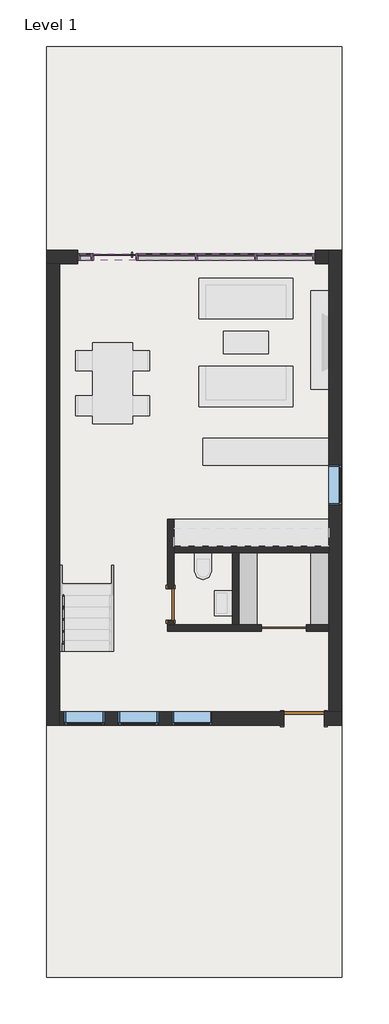
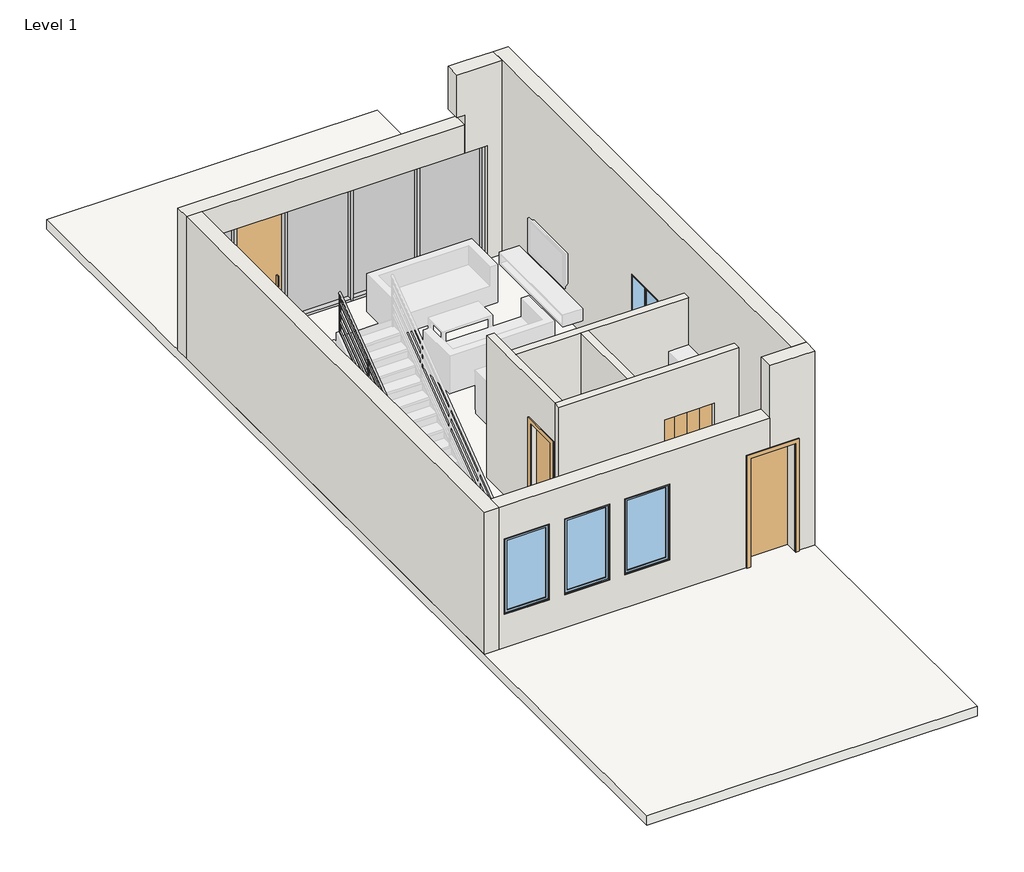
# One storey, part 1 of 2: 15 members, 10 walls, 4 doors, 4 plates, 4 windows, 1 railing, 1 slab.
"""IFC4 building model written with IfcOpenShell, lengths in millimetres."""

import ifcopenshell
import ifcopenshell.guid

model = None  # the IFC model being written
_history = None  # IfcOwnerHistory: only IFC2X3 demands one
_inside = {}  # id of a spatial element -> (the spatial element, [elements in it])
_under = {}  # id of a project, library or spatial element -> (it, [spatial elements below it])
_declared = {}  # id of a project -> (the project, [libraries it declares])
_typed = {}  # id of a type object -> (the type object, [elements of that type])
_made_of = {}  # id of a material, layer set ... -> (it, [elements and type objects made of it])


def new_model(schema):
    """Start an empty IFC model of exactly this schema.

    Asked for "IFC4X3", IfcOpenShell would pick the latest addendum, in which some entities
    have other attributes; the version numbers below select the first issue.
    IFC2X3 requires an IfcOwnerHistory on every rooted entity: one is made here for all.
    """
    global model, _history
    if schema == "IFC4X3":
        model = ifcopenshell.file(schema_version=(4, 3, 0, 0))
    else:
        model = ifcopenshell.file(schema=schema)
    _inside.clear()
    _under.clear()
    _declared.clear()
    _typed.clear()
    _made_of.clear()
    _history = None
    if model.schema == "IFC2X3":
        org = make("IfcOrganization", Name="unknown")
        user = make(
            "IfcPersonAndOrganization",
            ThePerson=make("IfcPerson", FamilyName="unknown"),
            TheOrganization=org,
        )
        app = make(
            "IfcApplication",
            ApplicationDeveloper=org,
            Version="unknown",
            ApplicationFullName="unknown",
            ApplicationIdentifier="unknown",
        )
        _history = make(
            "IfcOwnerHistory",
            OwningUser=user,
            OwningApplication=app,
            ChangeAction="ADDED",
            CreationDate=0,
        )
    return model


def make(cls, **values):
    """One entity of the class cls with the attributes given. An attribute that is None is left unset."""
    return model.create_entity(
        cls, **{name: value for name, value in values.items() if value is not None}
    )


def rooted(cls, **values):
    """An entity with a GlobalId (a new one), such as an element, a storey or a relation."""
    return make(cls, GlobalId=ifcopenshell.guid.new(), OwnerHistory=_history, **values)


def si_unit(unit_type, name, prefix=None):
    """IfcSIUnit, for example si_unit("LENGTHUNIT", "METRE", prefix="MILLI")."""
    return make("IfcSIUnit", UnitType=unit_type, Prefix=prefix, Name=name)


def assignment(units):
    """IfcUnitAssignment: the units of a project."""
    return None if units is None else make("IfcUnitAssignment", Units=units)


def point(xyz):
    """IfcCartesianPoint."""
    return None if xyz is None else make("IfcCartesianPoint", Coordinates=xyz)


def direction(xyz):
    """IfcDirection."""
    return None if xyz is None else make("IfcDirection", DirectionRatios=xyz)


def frame(location, z_axis=None, x_axis=None):
    """IfcAxis2Placement3D, a coordinate frame: its origin and axes. An axis left out is left unset."""
    return make(
        "IfcAxis2Placement3D",
        Location=point(location),
        Axis=direction(z_axis),
        RefDirection=direction(x_axis),
    )


def origin():
    """The frame at (0, 0, 0) with its axes left unset."""
    return frame((0.0, 0.0, 0.0))


def origin_with_axes():
    """The frame at (0, 0, 0) with the z axis (0, 0, 1) and the x axis (1, 0, 0) written out."""
    return frame((0.0, 0.0, 0.0), z_axis=(0.0, 0.0, 1.0), x_axis=(1.0, 0.0, 0.0))


def place(relative_to, where):
    """IfcLocalPlacement: puts the frame where relative to a parent placement (None: the world)."""
    return make(
        "IfcLocalPlacement", PlacementRelTo=relative_to, RelativePlacement=where
    )


def context(
    kind, dimensions, precision=None, world=None, true_north=None, identifier=None
):
    """IfcGeometricRepresentationContext, for example the 3D "Model" context."""
    return make(
        "IfcGeometricRepresentationContext",
        ContextIdentifier=identifier,
        ContextType=kind,
        CoordinateSpaceDimension=dimensions,
        Precision=precision,
        WorldCoordinateSystem=world,
        TrueNorth=true_north,
    )


def project(units=None, contexts=None):
    """IfcProject with its units and contexts."""
    return rooted(
        "IfcProject",
        Name="project",
        RepresentationContexts=contexts,
        UnitsInContext=assignment(units),
    )


def spatial(cls, under=None, at=None, **own):
    """A site, building, storey or space (cls), placed at a placement, below another one or the project."""
    s = rooted(cls, ObjectPlacement=at, **own)
    if under is not None:
        _under.setdefault(under.id(), (under, []))[1].append(s)
    return s


def polyline(points):
    """IfcPolyline through the points."""
    return make("IfcPolyline", Points=[point(p) for p in points])


def circle_curve(where, radius):
    """IfcCircle in the frame where."""
    return make("IfcCircle", Position=where, Radius=radius)


def ellipse_curve(where, semi_axis1, semi_axis2):
    """IfcEllipse in the frame where."""
    return make(
        "IfcEllipse", Position=where, SemiAxis1=semi_axis1, SemiAxis2=semi_axis2
    )


def outline(outer, holes=None, kind="AREA"):
    """IfcArbitraryClosedProfileDef: a profile drawn as a closed curve; with holes, ...WithVoids."""
    if holes is None:
        return make("IfcArbitraryClosedProfileDef", ProfileType=kind, OuterCurve=outer)
    return make(
        "IfcArbitraryProfileDefWithVoids",
        ProfileType=kind,
        OuterCurve=outer,
        InnerCurves=holes,
    )


def extrude(swept, where, along, depth):
    """IfcExtrudedAreaSolid: the profile swept, set in the frame where, extruded along a direction by depth."""
    return make(
        "IfcExtrudedAreaSolid",
        SweptArea=swept,
        Position=where,
        ExtrudedDirection=direction(along),
        Depth=depth,
    )


def faces_of(points, faces, orient=None, outer=None):
    """IfcFace entities. A face is a list of loops; a loop is a list of indices into points, from 0.

    orient and outer hold one flag for each loop. By default every Orientation is true, the
    first loop of a face is its IfcFaceOuterBound and the others are IfcFaceBound.
    """
    made = []
    for i, loops in enumerate(faces):
        bounds = []
        for j, loop in enumerate(loops):
            is_outer = j == 0 if outer is None else outer[i][j]
            bounds.append(
                make(
                    "IfcFaceOuterBound" if is_outer else "IfcFaceBound",
                    Bound=make("IfcPolyLoop", Polygon=[points[k] for k in loop]),
                    Orientation=True if orient is None else orient[i][j],
                )
            )
        made.append(make("IfcFace", Bounds=bounds))
    return made


def faceted_brep(points, faces, orient=None, outer=None, voids=None):
    """IfcFacetedBrep: a solid bounded by flat faces; with voids (closed shells), ...WithVoids."""
    shared = [point(p) for p in points]
    hull = make("IfcClosedShell", CfsFaces=faces_of(shared, faces, orient, outer))
    if voids is None:
        return make("IfcFacetedBrep", Outer=hull)
    return make(
        "IfcFacetedBrepWithVoids",
        Outer=hull,
        Voids=[
            make(cls, CfsFaces=faces_of(shared, fs, o, b)) for cls, fs, o, b in voids
        ],
    )


def shape(context_of_items, identifier, shape_type, items):
    """IfcShapeRepresentation: the items that make up one representation, for example the "Body"."""
    return make(
        "IfcShapeRepresentation",
        ContextOfItems=context_of_items,
        RepresentationIdentifier=identifier,
        RepresentationType=shape_type,
        Items=items,
    )


def source(mapping_origin, context_of_items, identifier, shape_type, items):
    """IfcRepresentationMap: a shape defined once, which mapped items show again and again."""
    return make(
        "IfcRepresentationMap",
        MappingOrigin=mapping_origin,
        MappedRepresentation=shape(context_of_items, identifier, shape_type, items),
    )


def transform(
    local_origin,
    x_axis=None,
    y_axis=None,
    z_axis=None,
    scale=None,
    scale2=None,
    scale3=None,
    uniform=True,
):
    """IfcCartesianTransformationOperator3D, or its non-uniform kind. x_axis, y_axis, z_axis: its Axis1, 2, 3."""
    if uniform:
        return make(
            "IfcCartesianTransformationOperator3D",
            Axis1=direction(x_axis),
            Axis2=direction(y_axis),
            LocalOrigin=point(local_origin),
            Scale=scale,
            Axis3=direction(z_axis),
        )
    return make(
        "IfcCartesianTransformationOperator3DnonUniform",
        Axis1=direction(x_axis),
        Axis2=direction(y_axis),
        LocalOrigin=point(local_origin),
        Scale=scale,
        Axis3=direction(z_axis),
        Scale2=scale2,
        Scale3=scale3,
    )


def mapped(mapping_source, mapping_target):
    """IfcMappedItem: shows the shape of a source again, moved by a transform."""
    return make(
        "IfcMappedItem", MappingSource=mapping_source, MappingTarget=mapping_target
    )


def made_of(thing, what):
    """Note that an element or type object is made of a material, layer set ...; save() writes the relation."""
    if what is not None:
        _made_of.setdefault(what.id(), (what, []))[1].append(thing)
    return thing


def element(
    cls,
    number,
    at=None,
    inside=None,
    cuts=None,
    type_object=None,
    material=None,
    context=None,
    identifier="Body",
    shape_type=None,
    held_by="IfcProductDefinitionShape",
    body=None,
    shapes=None,
    **own,
):
    """One element of the class cls, such as IfcWall. Its Tag is "e" and its number.

    at: its placement. inside: the storey or other place that contains it. cuts: it is an
    opening in that element (IfcRelVoidsElement). A single representation is given by context,
    identifier, shape_type and body (its items); several are given by shapes. held_by: the class
    of the entity that holds the representations. save() writes the other relations.
    """
    e = rooted(cls, Tag="e%d" % number, ObjectPlacement=at, **own)
    if body is not None:
        shapes = [shape(context, identifier, shape_type, body)]
    if shapes is not None:
        e.Representation = make(held_by, Representations=shapes)
    if inside is not None:
        _inside.setdefault(inside.id(), (inside, []))[1].append(e)
    if cuts is not None:
        rooted(
            "IfcRelVoidsElement", RelatingBuildingElement=cuts, RelatedOpeningElement=e
        )
    if type_object is not None:
        _typed.setdefault(type_object.id(), (type_object, []))[1].append(e)
    return made_of(e, material)


def aggregate(whole, parts):
    """IfcRelAggregates: a whole, such as a stair, and the parts it consists of."""
    return rooted("IfcRelAggregates", RelatingObject=whole, RelatedObjects=parts)


def save(model, path):
    """Write the relations noted so far, then the file.

    IfcRelAggregates (storeys below a building ...), IfcRelContainedInSpatialStructure (elements
    in a storey), IfcRelDefinesByType, IfcRelAssociatesMaterial and IfcRelDeclares: one each for
    every whole, place, type object, material and project.
    """
    for whole, parts in _under.values():
        aggregate(whole, parts)
    for where, things in _inside.values():
        rooted(
            "IfcRelContainedInSpatialStructure",
            RelatedElements=things,
            RelatingStructure=where,
        )
    for kind, things in _typed.values():
        rooted("IfcRelDefinesByType", RelatedObjects=things, RelatingType=kind)
    for what, things in _made_of.values():
        rooted("IfcRelAssociatesMaterial", RelatedObjects=things, RelatingMaterial=what)
    for by, libraries in _declared.values():
        rooted("IfcRelDeclares", RelatingContext=by, RelatedDefinitions=libraries)
    model.write(path)


def plane_surface(at):
    """IfcPlane: the flat surface through the origin of the frame at, square to its z axis."""
    return make("IfcPlane", Position=at)


def cylinder_surface(at, radius):
    """IfcCylindricalSurface: all points at the distance radius from the z axis of the frame at."""
    return make("IfcCylindricalSurface", Position=at, Radius=radius)


def advanced_brep(points, edges, surfaces, faces):
    """IfcAdvancedBrep: a solid bounded by faces that lie on surfaces and meet in shared edges.

    An edge is (start, end): straight between two places in points (the first is 0);
    or (start, end, curve); or (start, end, curve, False) where it runs against its curve.
    A face is (place in surfaces, loops), or (place, loops, False) where it looks against
    its surface's normal. A loop lists edges by number (the first is 1), with a minus sign
    where the edge is run from its end to its start. The first loop is the outer one.
    """
    corners = [point(p) for p in points]
    vertices = [make("IfcVertexPoint", VertexGeometry=c) for c in corners]
    made = []
    for start, end, *more in edges:
        made.append(
            make(
                "IfcEdgeCurve",
                EdgeStart=vertices[start],
                EdgeEnd=vertices[end],
                EdgeGeometry=more[0] if more else make("IfcPolyline", Points=[corners[start], corners[end]]),
                SameSense=more[1] if len(more) > 1 else True,
            )
        )
    hull = []
    for where, loops, *sense in faces:
        bounds = []
        for j, loop in enumerate(loops):
            ring = [make("IfcOrientedEdge", EdgeElement=made[abs(k) - 1], Orientation=k > 0) for k in loop]
            bounds.append(
                make(
                    "IfcFaceOuterBound" if j == 0 else "IfcFaceBound",
                    Bound=make("IfcEdgeLoop", EdgeList=ring),
                    Orientation=True,
                )
            )
        hull.append(make("IfcAdvancedFace", Bounds=bounds, FaceSurface=surfaces[where], SameSense=sense[0] if sense else True))
    return make("IfcAdvancedBrep", Outer=make("IfcClosedShell", CfsFaces=hull))


def door_88445510(model_context):
    return source(origin(), model_context, "Body", "SweptSolid", [
        extrude(outline(polyline([(255.0, 10.0), (500.0, 10.0), (500.0, -10.0), (-500.0, -10.0), (-500.0, 10.0), (-255.0, 10.0), (-255.0, 0.0), (-245.0, 0.0), (-245.0, 10.0), (-5.0, 10.0), (-5.0, 0.0), (5.0, 0.0), (5.0, 10.0), (245.0, 10.0), (245.0, 0.0), (255.0, 0.0), (255.0, 10.0)])), origin_with_axes(), (0.0, 0.0, 1.0), 2000.0),
    ])


def ba_basic_door_70_x_210cm_b6d038f8(model_context):
    return source(origin(), model_context, "Body", "SweptSolid", [
        extrude(outline(polyline([(350.0, 24.0), (-350.0, 24.0), (-350.0, 75.0), (350.0, 75.0), (350.0, 24.0)])), origin_with_axes(), (0.0, 0.0, 1.0), 2100.0),
        extrude(outline(polyline([(2176.0, -426.0), (0.0, -426.0), (0.0, -350.0), (2100.0, -350.0), (2100.0, 350.0), (0.0, 350.0), (0.0, 426.0), (2176.0, 426.0), (2176.0, -426.0)])), frame((0.0, 75.0, 0.0), z_axis=(0.0, 1.0, 0.0), x_axis=(0.0, 0.0, 1.0)), (0.0, 0.0, 1.0), 25.0),
        extrude(outline(polyline([(2176.0, 426.0), (2176.0, -426.0), (0.0, -426.0), (0.0, -350.0), (2100.0, -350.0), (2100.0, 350.0), (0.0, 350.0), (0.0, 426.0), (2176.0, 426.0)])), frame((0.0, -100.0, 0.0), z_axis=(0.0, 1.0, 0.0), x_axis=(0.0, 0.0, 1.0)), (0.0, 0.0, 1.0), 25.0),
    ])


def ba_basic_door_90_x_230cm_e5931120(model_context):
    return source(origin(), model_context, "Body", "SweptSolid", [
        extrude(outline(polyline([(450.0, 99.0), (-450.0, 99.0), (-450.0, 150.0), (450.0, 150.0), (450.0, 99.0)])), origin_with_axes(), (0.0, 0.0, 1.0), 2300.0),
        extrude(outline(polyline([(2376.0, -526.0), (0.0, -526.0), (0.0, -450.0), (2300.0, -450.0), (2300.0, 450.0), (0.0, 450.0), (0.0, 526.0), (2376.0, 526.0), (2376.0, -526.0)])), frame((0.0, 150.0, 0.0), z_axis=(0.0, 1.0, 0.0), x_axis=(0.0, 0.0, 1.0)), (0.0, 0.0, 1.0), 25.0),
        extrude(outline(polyline([(2376.0, 526.0), (2376.0, -526.0), (0.0, -526.0), (0.0, -450.0), (2300.0, -450.0), (2300.0, 450.0), (0.0, 450.0), (0.0, 526.0), (2376.0, 526.0)])), frame((0.0, -175.0, 0.0), z_axis=(0.0, 1.0, 0.0), x_axis=(0.0, 0.0, 1.0)), (0.0, 0.0, 1.0), 25.0),
    ])


def m_door_curtain_wall_single_glass_m_door_curtain_wall_single_99f07895(model_context):
    return source(origin(), model_context, "Body", "SweptSolid", [
        extrude(outline(polyline([(475.0, -50.8), (-475.0, -50.8), (-475.0, -38.1), (475.0, -38.1), (475.0, -50.8)])), origin_with_axes(), (0.0, 0.0, 1.0), 2350.0),
        extrude(outline(polyline([(-373.4, 12.7), (-373.4, -38.1), (-398.8, -38.1), (-398.8, 12.7), (-373.4, 12.7)])), frame((0.0, 0.0, 762.0), z_axis=(0.0, 0.0, 1.0), x_axis=(1.0, 0.0, 0.0)), (0.0, 0.0, 1.0), 228.6),
        extrude(outline(polyline([(-398.8, -101.6), (-398.8, -50.8), (-373.4, -50.8), (-373.4, -101.6), (-398.8, -101.6)])), frame((0.0, 0.0, 762.0), z_axis=(0.0, 0.0, 1.0), x_axis=(1.0, 0.0, 0.0)), (0.0, 0.0, 1.0), 228.6),
    ])


def rectangular_mullion_50_x_150mm_8d7ec0e8(model_context):
    return source(origin(), model_context, "Body", "SweptSolid", [
        extrude(outline(polyline([(0.0, 75.0), (0.0, -75.0), (-50.0, -75.0), (-50.0, 75.0), (0.0, 75.0)])), frame((0.0, 0.0, -1250.0000002), z_axis=(0.0, 0.0, 1.0), x_axis=(1.0, 0.0, 0.0)), (0.0, 0.0, 1.0), 1250.0000002),
    ])


def rectangular_mullion_50_x_150mm_345eee08(model_context):
    return source(origin(), model_context, "Body", "SweptSolid", [
        extrude(outline(polyline([(0.0, 75.0), (0.0, -75.0), (-50.0, -75.0), (-50.0, 75.0), (0.0, 75.0)])), frame((0.0, 0.0, -1274.9999998), z_axis=(0.0, 0.0, 1.0), x_axis=(1.0, 0.0, 0.0)), (0.0, 0.0, 1.0), 1274.9999998),
    ])


def rectangular_mullion_50_x_150mm_6225e4e3(model_context):
    return source(origin(), model_context, "Body", "SweptSolid", [
        extrude(outline(polyline([(25.0, 75.0), (25.0, -75.0), (-25.0, -75.0), (-25.0, 75.0), (25.0, 75.0)])), frame((0.0, 0.0, -2400.0), z_axis=(0.0, 0.0, 1.0), x_axis=(1.0, 0.0, 0.0)), (0.0, 0.0, 1.0), 2400.0),
    ])


def rectangular_mullion_50_x_150mm_662c37b1(model_context):
    return source(origin(), model_context, "Body", "SweptSolid", [
        extrude(outline(polyline([(0.0, 75.0), (0.0, -75.0), (-50.0, -75.0), (-50.0, 75.0), (0.0, 75.0)])), frame((0.0, 0.0, -2400.0), z_axis=(0.0, 0.0, 1.0), x_axis=(1.0, 0.0, 0.0)), (0.0, 0.0, 1.0), 2400.0),
    ])


def rectangular_mullion_50_x_150mm_12a430f9(model_context):
    return source(origin(), model_context, "Body", "SweptSolid", [
        extrude(outline(polyline([(0.0, 75.0), (0.0, -75.0), (-50.0, -75.0), (-50.0, 75.0), (0.0, 75.0)])), frame((0.0, 0.0, -950.0), z_axis=(0.0, 0.0, 1.0), x_axis=(1.0, 0.0, 0.0)), (0.0, 0.0, 1.0), 950.0),
    ])


def rectangular_mullion_50_x_150mm_43431b2b(model_context):
    return source(origin(), model_context, "Body", "SweptSolid", [
        extrude(outline(polyline([(0.0, 75.0), (0.0, -75.0), (-50.0, -75.0), (-50.0, 75.0), (0.0, 75.0)])), frame((0.0, 0.0, -250.0000002), z_axis=(0.0, 0.0, 1.0), x_axis=(1.0, 0.0, 0.0)), (0.0, 0.0, 1.0), 250.0000002),
    ])


def system_panel_glazed_960e6087(model_context):
    return source(origin(), model_context, "Body", "SweptSolid", [
        extrude(outline(polyline([(625.0000001, 24.5), (-625.0000001, 24.5), (-625.0000001, 49.5), (625.0000001, 49.5), (625.0000001, 24.5)])), origin_with_axes(), (0.0, 0.0, 1.0), 2300.0),
    ])


def system_panel_glazed_939e179a(model_context):
    return source(origin(), model_context, "Body", "SweptSolid", [
        extrude(outline(polyline([(637.4999999, 24.5), (-637.4999999, 24.5), (-637.4999999, 49.5), (637.4999999, 49.5), (637.4999999, 24.5)])), origin_with_axes(), (0.0, 0.0, 1.0), 2300.0),
    ])


def system_panel_glazed_27ab1db5(model_context):
    return source(origin(), model_context, "Body", "SweptSolid", [
        extrude(outline(polyline([(125.0000001, 24.5), (-125.0000001, 24.5), (-125.0000001, 49.5), (125.0000001, 49.5), (125.0000001, 24.5)])), origin_with_axes(), (0.0, 0.0, 1.0), 2300.0),
    ])


def ba_window_900_x_1600mm_2_0de2e490(model_context):
    return source(origin(), model_context, "Body", "SweptSolid", [
        extrude(outline(polyline([(-387.0, 128.0), (387.0, 128.0), (387.0, 116.0), (-387.0, 116.0), (-387.0, 128.0)])), frame((0.0, 0.0, 978.0), z_axis=(0.0, 0.0, 1.0), x_axis=(1.0, 0.0, 0.0)), (0.0, 0.0, 1.0), 1474.0),
        extrude(outline(polyline([(2496.0, -431.0), (934.0, -431.0), (934.0, 431.0), (2496.0, 431.0), (2496.0, -431.0)]), holes=[polyline([(2452.0, -387.0), (2452.0, 387.0), (978.0, 387.0), (978.0, -387.0), (2452.0, -387.0)])]), frame((0.0, 100.0, 0.0), z_axis=(0.0, 1.0, 0.0), x_axis=(0.0, 0.0, 1.0)), (0.0, 0.0, 1.0), 44.0),
        extrude(outline(polyline([(2515.0, -450.0), (915.0, -450.0), (915.0, 450.0), (2515.0, 450.0), (2515.0, -450.0)]), holes=[polyline([(2496.0, -431.0), (2496.0, 431.0), (934.0, 431.0), (934.0, -431.0), (2496.0, -431.0)])]), frame((0.0, 100.0, 0.0), z_axis=(0.0, 1.0, 0.0), x_axis=(0.0, 0.0, 1.0)), (0.0, 0.0, 1.0), 63.0),
        extrude(outline(polyline([(2515.0, -450.0), (915.0, -450.0), (915.0, 450.0), (2515.0, 450.0), (2515.0, -450.0)]), holes=[polyline([(2483.0, -418.0), (2483.0, 418.0), (947.0, 418.0), (947.0, -418.0), (2483.0, -418.0)])]), frame((0.0, -137.0, 0.0), z_axis=(0.0, 1.0, 0.0), x_axis=(0.0, 0.0, 1.0)), (0.0, 0.0, 1.0), 237.0),
    ])


def ba_window_900_x_1600mm_2_f3ed7943(model_context):
    return source(origin(), model_context, "Body", "SweptSolid", [
        extrude(outline(polyline([(-387.0, -128.0), (-387.0, -116.0), (387.0, -116.0), (387.0, -128.0), (-387.0, -128.0)])), frame((0.0, 0.0, 978.0), z_axis=(0.0, 0.0, 1.0), x_axis=(1.0, 0.0, 0.0)), (0.0, 0.0, 1.0), 1474.0),
        extrude(outline(polyline([(2496.0, -431.0), (934.0, -431.0), (934.0, 431.0), (2496.0, 431.0), (2496.0, -431.0)]), holes=[polyline([(2452.0, -387.0), (2452.0, 387.0), (978.0, 387.0), (978.0, -387.0), (2452.0, -387.0)])]), frame((0.0, -144.0, 0.0), z_axis=(0.0, 1.0, 0.0), x_axis=(0.0, 0.0, 1.0)), (0.0, 0.0, 1.0), 44.0),
        extrude(outline(polyline([(2515.0, -450.0), (915.0, -450.0), (915.0, 450.0), (2515.0, 450.0), (2515.0, -450.0)]), holes=[polyline([(2496.0, -431.0), (2496.0, 431.0), (934.0, 431.0), (934.0, -431.0), (2496.0, -431.0)])]), frame((0.0, -163.0, 0.0), z_axis=(0.0, 1.0, 0.0), x_axis=(0.0, 0.0, 1.0)), (0.0, 0.0, 1.0), 63.0),
        extrude(outline(polyline([(2515.0, -450.0), (915.0, -450.0), (915.0, 450.0), (2515.0, 450.0), (2515.0, -450.0)]), holes=[polyline([(2483.0, -418.0), (2483.0, 418.0), (947.0, 418.0), (947.0, -418.0), (2483.0, -418.0)])]), frame((0.0, -100.0, 0.0), z_axis=(0.0, 1.0, 0.0), x_axis=(0.0, 0.0, 1.0)), (0.0, 0.0, 1.0), 237.0),
    ])


model = new_model("IFC4")

# Units and contexts
model_context = context("Model", 3, world=origin())
ifc_project = project(units=[si_unit("LENGTHUNIT", "METRE", prefix="MILLI")], contexts=[model_context])

# Site, building, storey
site = spatial("IfcSite", under=ifc_project)
building = spatial("IfcBuilding", under=site)
storey = spatial("IfcBuildingStorey", under=building, Name="Level 1", Elevation=0.0)

# Doors
placement = place(None, origin())
door_shape = door_88445510(model_context)
element("IfcDoor", 1, ObjectType="BA_Bi-fold door : AD_Bi-fold door - 100cm", at=placement, inside=storey, context=model_context, shape_type="MappedRepresentation", body=[
    mapped(door_shape, transform((2017.9856921, -6579.202269, 0.0), x_axis=(-1.0, 0.0, 0.0), y_axis=(0.0, -1.0, 0.0), z_axis=(0.0, 0.0, 1.0))),
])
ba_basic_door_70_x_210cm_shape = ba_basic_door_70_x_210cm_b6d038f8(model_context)
element("IfcDoor", 2, ObjectType="BA_Basic Door : 70 x 210cm", at=placement, inside=storey, context=model_context, shape_type="MappedRepresentation", body=[
    mapped(ba_basic_door_70_x_210cm_shape, transform((-507.0143079, -6054.202269, 0.0), x_axis=(0.0, -1.0, 0.0), y_axis=(1.0, 0.0, 0.0), z_axis=(0.0, 0.0, 1.0))),
])
ba_basic_door_90_x_230cm_shape = ba_basic_door_90_x_230cm_e5931120(model_context)
element("IfcDoor", 3, ObjectType="BA_Basic Door : 90 x 230cm", at=placement, inside=storey, context=model_context, shape_type="MappedRepresentation", body=[
    mapped(ba_basic_door_90_x_230cm_shape, transform((2467.9856921, -8604.202269, 0.0), x_axis=(1.0, 0.0, 0.0), y_axis=(0.0, 1.0, 0.0), z_axis=(0.0, 0.0, 1.0))),
])
m_door_curtain_wall_single_glass_m_door_curtain_wall_single_shape = m_door_curtain_wall_single_glass_m_door_curtain_wall_single_99f07895(model_context)
element("IfcDoor", 4, ObjectType="M_Door-Curtain-Wall-Single-Glass : M_Door-Curtain-Wall-Single-Glass", at=placement, inside=storey, context=model_context, shape_type="MappedRepresentation", body=[
    mapped(m_door_curtain_wall_single_glass_m_door_curtain_wall_single_shape, transform((-1757.0143078, 1695.797731, 0.0), x_axis=(-1.0, 0.0, 0.0), y_axis=(0.0, -1.0, 0.0), z_axis=(0.0, 0.0, 1.0))),
])

# Members
rectangular_mullion_50_x_150mm_shape = rectangular_mullion_50_x_150mm_8d7ec0e8(model_context)
element("IfcMember", 5, ObjectType="Rectangular Mullion : 50 x 150mm", at=placement, inside=storey, context=model_context, shape_type="MappedRepresentation", body=[
    mapped(rectangular_mullion_50_x_150mm_shape, transform((2667.9856921, 1695.797731, 2400.0), x_axis=(0.0, 0.0, 1.0), y_axis=(0.0, -1.0, 0.0), z_axis=(1.0, 0.0, 0.0))),
])
rectangular_mullion_50_x_150mm_2_shape = rectangular_mullion_50_x_150mm_345eee08(model_context)
element("IfcMember", 6, ObjectType="Rectangular Mullion : 50 x 150mm", at=placement, inside=storey, context=model_context, shape_type="MappedRepresentation", body=[
    mapped(rectangular_mullion_50_x_150mm_2_shape, transform((42.9856921, 1695.797731, 2400.0), x_axis=(0.0, 0.0, 1.0), y_axis=(0.0, -1.0, 0.0), z_axis=(1.0, 0.0, 0.0))),
])
element("IfcMember", 7, ObjectType="Rectangular Mullion : 50 x 150mm", at=placement, inside=storey, context=model_context, shape_type="MappedRepresentation", body=[
    mapped(rectangular_mullion_50_x_150mm_2_shape, transform((1367.9856919, 1695.797731, 2400.0), x_axis=(0.0, 0.0, 1.0), y_axis=(0.0, -1.0, 0.0), z_axis=(1.0, 0.0, 0.0))),
])
element("IfcMember", 8, ObjectType="Rectangular Mullion : 50 x 150mm", at=placement, inside=storey, context=model_context, shape_type="MappedRepresentation", body=[
    mapped(rectangular_mullion_50_x_150mm_shape, transform((1417.9856919, 1695.797731, 0.0), x_axis=(0.0, 0.0, -1.0), y_axis=(0.0, -1.0, 0.0), z_axis=(-1.0, 0.0, 0.0))),
])
element("IfcMember", 9, ObjectType="Rectangular Mullion : 50 x 150mm", at=placement, inside=storey, context=model_context, shape_type="MappedRepresentation", body=[
    mapped(rectangular_mullion_50_x_150mm_2_shape, transform((-1232.0143078, 1695.797731, 0.0), x_axis=(0.0, 0.0, -1.0), y_axis=(0.0, -1.0, 0.0), z_axis=(-1.0, 0.0, 0.0))),
])
element("IfcMember", 10, ObjectType="Rectangular Mullion : 50 x 150mm", at=placement, inside=storey, context=model_context, shape_type="MappedRepresentation", body=[
    mapped(rectangular_mullion_50_x_150mm_2_shape, transform((92.9856921, 1695.797731, 0.0), x_axis=(0.0, 0.0, -1.0), y_axis=(0.0, -1.0, 0.0), z_axis=(-1.0, 0.0, 0.0))),
])
rectangular_mullion_50_x_150mm_3_shape = rectangular_mullion_50_x_150mm_6225e4e3(model_context)
element("IfcMember", 11, ObjectType="Rectangular Mullion : 50 x 150mm", at=placement, inside=storey, context=model_context, shape_type="MappedRepresentation", body=[
    mapped(rectangular_mullion_50_x_150mm_3_shape, transform((-1257.0143078, 1695.797731, 0.0), x_axis=(1.0, 0.0, 0.0), y_axis=(0.0, -1.0, 0.0), z_axis=(0.0, 0.0, -1.0))),
])
element("IfcMember", 12, ObjectType="Rectangular Mullion : 50 x 150mm", at=placement, inside=storey, context=model_context, shape_type="MappedRepresentation", body=[
    mapped(rectangular_mullion_50_x_150mm_3_shape, transform((67.9856921, 1695.797731, 0.0), x_axis=(1.0, 0.0, 0.0), y_axis=(0.0, -1.0, 0.0), z_axis=(0.0, 0.0, -1.0))),
])
element("IfcMember", 13, ObjectType="Rectangular Mullion : 50 x 150mm", at=placement, inside=storey, context=model_context, shape_type="MappedRepresentation", body=[
    mapped(rectangular_mullion_50_x_150mm_3_shape, transform((1392.9856919, 1695.797731, 0.0), x_axis=(1.0, 0.0, 0.0), y_axis=(0.0, -1.0, 0.0), z_axis=(0.0, 0.0, -1.0))),
])
element("IfcMember", 14, ObjectType="Rectangular Mullion : 50 x 150mm", at=placement, inside=storey, context=model_context, shape_type="MappedRepresentation", body=[
    mapped(rectangular_mullion_50_x_150mm_3_shape, transform((-2257.0143078, 1695.797731, 0.0), x_axis=(1.0, 0.0, 0.0), y_axis=(0.0, -1.0, 0.0), z_axis=(0.0, 0.0, -1.0))),
])
rectangular_mullion_50_x_150mm_4_shape = rectangular_mullion_50_x_150mm_662c37b1(model_context)
element("IfcMember", 15, ObjectType="Rectangular Mullion : 50 x 150mm", at=placement, inside=storey, context=model_context, shape_type="MappedRepresentation", body=[
    mapped(rectangular_mullion_50_x_150mm_4_shape, transform((2717.9856921, 1695.797731, 0.0), x_axis=(1.0, 0.0, 0.0), y_axis=(0.0, -1.0, 0.0), z_axis=(0.0, 0.0, -1.0))),
])
element("IfcMember", 16, ObjectType="Rectangular Mullion : 50 x 150mm", at=placement, inside=storey, context=model_context, shape_type="MappedRepresentation", body=[
    mapped(rectangular_mullion_50_x_150mm_4_shape, transform((-2582.0143079, 1695.797731, 2400.0), x_axis=(-1.0, 0.0, 0.0), y_axis=(0.0, -1.0, 0.0), z_axis=(0.0, 0.0, 1.0))),
])
rectangular_mullion_50_x_150mm_5_shape = rectangular_mullion_50_x_150mm_12a430f9(model_context)
element("IfcMember", 17, ObjectType="Rectangular Mullion : 50 x 150mm", at=placement, inside=storey, context=model_context, shape_type="MappedRepresentation", body=[
    mapped(rectangular_mullion_50_x_150mm_5_shape, transform((-1282.0143078, 1695.797731, 2400.0), x_axis=(0.0, 0.0, 1.0), y_axis=(0.0, -1.0, 0.0), z_axis=(1.0, 0.0, 0.0))),
])
rectangular_mullion_50_x_150mm_6_shape = rectangular_mullion_50_x_150mm_43431b2b(model_context)
element("IfcMember", 18, ObjectType="Rectangular Mullion : 50 x 150mm", at=placement, inside=storey, context=model_context, shape_type="MappedRepresentation", body=[
    mapped(rectangular_mullion_50_x_150mm_6_shape, transform((-2532.0143079, 1695.797731, 0.0), x_axis=(0.0, 0.0, -1.0), y_axis=(0.0, -1.0, 0.0), z_axis=(-1.0, 0.0, 0.0))),
])
element("IfcMember", 19, ObjectType="Rectangular Mullion : 50 x 150mm", at=placement, inside=storey, context=model_context, shape_type="MappedRepresentation", body=[
    mapped(rectangular_mullion_50_x_150mm_6_shape, transform((-2282.0143078, 1695.797731, 2400.0), x_axis=(0.0, 0.0, 1.0), y_axis=(0.0, -1.0, 0.0), z_axis=(1.0, 0.0, 0.0))),
])

# Plates
system_panel_glazed_shape = system_panel_glazed_960e6087(model_context)
element("IfcPlate", 20, ObjectType="System Panel : Glazed", at=placement, inside=storey, context=model_context, shape_type="MappedRepresentation", body=[
    mapped(system_panel_glazed_shape, transform((2042.985692, 1695.797731, 50.0), x_axis=(1.0, 0.0, 0.0), y_axis=(0.0, 1.0, 0.0), z_axis=(0.0, 0.0, 1.0))),
])
system_panel_glazed_2_shape = system_panel_glazed_939e179a(model_context)
element("IfcPlate", 21, ObjectType="System Panel : Glazed", at=placement, inside=storey, context=model_context, shape_type="MappedRepresentation", body=[
    mapped(system_panel_glazed_2_shape, transform((-594.5143079, 1695.797731, 50.0), x_axis=(1.0, 0.0, 0.0), y_axis=(0.0, 1.0, 0.0), z_axis=(0.0, 0.0, 1.0))),
])
element("IfcPlate", 22, ObjectType="System Panel : Glazed", at=placement, inside=storey, context=model_context, shape_type="MappedRepresentation", body=[
    mapped(system_panel_glazed_2_shape, transform((730.485692, 1695.797731, 50.0), x_axis=(1.0, 0.0, 0.0), y_axis=(0.0, 1.0, 0.0), z_axis=(0.0, 0.0, 1.0))),
])
system_panel_glazed_3_shape = system_panel_glazed_27ab1db5(model_context)
element("IfcPlate", 23, ObjectType="System Panel : Glazed", at=placement, inside=storey, context=model_context, shape_type="MappedRepresentation", body=[
    mapped(system_panel_glazed_3_shape, transform((-2407.0143079, 1695.797731, 50.0), x_axis=(1.0, 0.0, 0.0), y_axis=(0.0, 1.0, 0.0), z_axis=(0.0, 0.0, 1.0))),
])

# Railing
element("IfcRailing", 24, ObjectType="900mm Pipe", at=placement, inside=storey, context=model_context, shape_type="AdvancedBrep", body=[
    advanced_brep(
    [(-2886.6143079, -7104.202269, 1063.1999558), (-2926.6143079, -7104.202269, 1063.1999558), (-2886.6143079, -3104.202269, 4074.9646617), (-2926.6143079, -3104.202269, 4074.9646617)],
    [
        (0, 1, ellipse_curve(frame((-2906.6143079, -7104.202269, 1063.1999558), z_axis=(0.0, -1.0, 0.0), x_axis=(0.0, 0.0, -1.0)), 25.0353383, 20.0)),
        (1, 0, ellipse_curve(frame((-2906.6143079, -7104.202269, 1063.1999558), z_axis=(0.0, -1.0, 0.0), x_axis=(0.0, 0.0, -1.0)), 25.0353383, 20.0)),
        (2, 3, ellipse_curve(frame((-2906.6143079, -3104.202269, 4074.9646617), z_axis=(0.0, 1.0, 0.0), x_axis=(0.0, 0.0, -1.0)), 25.0353383, 20.0)),
        (3, 2, ellipse_curve(frame((-2906.6143079, -3104.202269, 4074.9646617), z_axis=(0.0, 1.0, 0.0), x_axis=(0.0, 0.0, -1.0)), 25.0353383, 20.0)),
        (0, 2),
        (3, 1),
    ],
    [
        plane_surface(frame((-2906.6143079, -7104.202269, 1088.2352941), z_axis=(0.0, -1.0, 0.0), x_axis=(0.0, 0.0, 1.0))),
        plane_surface(frame((-2906.6143079, -3104.202269, 4100.0), z_axis=(0.0, 1.0, 0.0), x_axis=(0.0, 0.0, 1.0))),
        cylinder_surface(frame((-2906.6143079, -7092.1722151, 1072.2578787), z_axis=(0.0, -0.7988707691396074, -0.6015026967639399), x_axis=(-1.0, 0.0, 0.0)), 20.0),
    ],
    [
        (0, [[1, 2]]),
        (1, [[3, 4]]),
        (2, [[-1, 5, -4, 6]]),
        (2, [[-2, -6, -3, -5]]),
    ],
),
    advanced_brep(
    [(-2891.6143079, -7104.202269, 869.4587904), (-2921.6143079, -7104.202269, 869.4587904), (-2891.6143079, -3104.202269, 3881.2234962), (-2921.6143079, -3104.202269, 3881.2234962)],
    [
        (0, 1, ellipse_curve(frame((-2906.6143079, -7104.202269, 869.4587904), z_axis=(0.0, -1.0, 0.0), x_axis=(0.0, 0.0, -1.0)), 18.7765038, 15.0)),
        (1, 0, ellipse_curve(frame((-2906.6143079, -7104.202269, 869.4587904), z_axis=(0.0, -1.0, 0.0), x_axis=(0.0, 0.0, -1.0)), 18.7765038, 15.0)),
        (2, 3, ellipse_curve(frame((-2906.6143079, -3104.202269, 3881.2234962), z_axis=(0.0, 1.0, 0.0), x_axis=(0.0, 0.0, -1.0)), 18.7765038, 15.0)),
        (3, 2, ellipse_curve(frame((-2906.6143079, -3104.202269, 3881.2234962), z_axis=(0.0, 1.0, 0.0), x_axis=(0.0, 0.0, -1.0)), 18.7765038, 15.0)),
        (0, 2),
        (3, 1),
    ],
    [
        plane_surface(frame((-2906.6143079, -7104.202269, 888.2352941), z_axis=(0.0, -1.0, 0.0), x_axis=(0.0, 0.0, 1.0))),
        plane_surface(frame((-2906.6143079, -3104.202269, 3900.0), z_axis=(0.0, 1.0, 0.0), x_axis=(0.0, 0.0, 1.0))),
        cylinder_surface(frame((-2906.6143079, -7095.1797286, 876.2522326), z_axis=(0.0, -0.7988707691396074, -0.6015026967639399), x_axis=(-1.0, 0.0, 0.0)), 15.0),
    ],
    [
        (0, [[1, 2]]),
        (1, [[3, 4]]),
        (2, [[-1, 5, -4, 6]]),
        (2, [[-2, -6, -3, -5]]),
    ],
),
    advanced_brep(
    [(-2891.6143079, -7104.202269, 669.4587904), (-2921.6143079, -7104.202269, 669.4587904), (-2891.6143079, -3104.202269, 3681.2234962), (-2921.6143079, -3104.202269, 3681.2234962)],
    [
        (0, 1, ellipse_curve(frame((-2906.6143079, -7104.202269, 669.4587904), z_axis=(0.0, -1.0, 0.0), x_axis=(0.0, 0.0, -1.0)), 18.7765038, 15.0)),
        (1, 0, ellipse_curve(frame((-2906.6143079, -7104.202269, 669.4587904), z_axis=(0.0, -1.0, 0.0), x_axis=(0.0, 0.0, -1.0)), 18.7765038, 15.0)),
        (2, 3, ellipse_curve(frame((-2906.6143079, -3104.202269, 3681.2234962), z_axis=(0.0, 1.0, 0.0), x_axis=(0.0, 0.0, -1.0)), 18.7765038, 15.0)),
        (3, 2, ellipse_curve(frame((-2906.6143079, -3104.202269, 3681.2234962), z_axis=(0.0, 1.0, 0.0), x_axis=(0.0, 0.0, -1.0)), 18.7765038, 15.0)),
        (0, 2),
        (3, 1),
    ],
    [
        plane_surface(frame((-2906.6143079, -7104.202269, 688.2352941), z_axis=(0.0, -1.0, 0.0), x_axis=(0.0, 0.0, 1.0))),
        plane_surface(frame((-2906.6143079, -3104.202269, 3700.0), z_axis=(0.0, 1.0, 0.0), x_axis=(0.0, 0.0, 1.0))),
        cylinder_surface(frame((-2906.6143079, -7095.1797286, 676.2522326), z_axis=(0.0, -0.7988707691396074, -0.6015026967639399), x_axis=(-1.0, 0.0, 0.0)), 15.0),
    ],
    [
        (0, [[1, 2]]),
        (1, [[3, 4]]),
        (2, [[-1, 5, -4, 6]]),
        (2, [[-2, -6, -3, -5]]),
    ],
),
    advanced_brep(
    [(-2891.6143079, -7104.202269, 469.4587904), (-2921.6143079, -7104.202269, 469.4587904), (-2891.6143079, -3104.202269, 3481.2234962), (-2921.6143079, -3104.202269, 3481.2234962)],
    [
        (0, 1, ellipse_curve(frame((-2906.6143079, -7104.202269, 469.4587904), z_axis=(0.0, -1.0, 0.0), x_axis=(0.0, 0.0, -1.0)), 18.7765038, 15.0)),
        (1, 0, ellipse_curve(frame((-2906.6143079, -7104.202269, 469.4587904), z_axis=(0.0, -1.0, 0.0), x_axis=(0.0, 0.0, -1.0)), 18.7765038, 15.0)),
        (2, 3, ellipse_curve(frame((-2906.6143079, -3104.202269, 3481.2234962), z_axis=(0.0, 1.0, 0.0), x_axis=(0.0, 0.0, -1.0)), 18.7765038, 15.0)),
        (3, 2, ellipse_curve(frame((-2906.6143079, -3104.202269, 3481.2234962), z_axis=(0.0, 1.0, 0.0), x_axis=(0.0, 0.0, -1.0)), 18.7765038, 15.0)),
        (0, 2),
        (3, 1),
    ],
    [
        plane_surface(frame((-2906.6143079, -7104.202269, 488.2352941), z_axis=(0.0, -1.0, 0.0), x_axis=(0.0, 0.0, 1.0))),
        plane_surface(frame((-2906.6143079, -3104.202269, 3500.0), z_axis=(0.0, 1.0, 0.0), x_axis=(0.0, 0.0, 1.0))),
        cylinder_surface(frame((-2906.6143079, -7095.1797286, 476.2522326), z_axis=(0.0, -0.7988707691396074, -0.6015026967639399), x_axis=(-1.0, 0.0, 0.0)), 15.0),
    ],
    [
        (0, [[1, 2]]),
        (1, [[3, 4]]),
        (2, [[-1, 5, -4, 6]]),
        (2, [[-2, -6, -3, -5]]),
    ],
),
    advanced_brep(
    [(-2891.6143079, -7104.202269, 269.4587904), (-2921.6143079, -7104.202269, 269.4587904), (-2891.6143079, -3104.202269, 3281.2234962), (-2921.6143079, -3104.202269, 3281.2234962)],
    [
        (0, 1, ellipse_curve(frame((-2906.6143079, -7104.202269, 269.4587904), z_axis=(0.0, -1.0, 0.0), x_axis=(0.0, 0.0, -1.0)), 18.7765038, 15.0)),
        (1, 0, ellipse_curve(frame((-2906.6143079, -7104.202269, 269.4587904), z_axis=(0.0, -1.0, 0.0), x_axis=(0.0, 0.0, -1.0)), 18.7765038, 15.0)),
        (2, 3, ellipse_curve(frame((-2906.6143079, -3104.202269, 3281.2234962), z_axis=(0.0, 1.0, 0.0), x_axis=(0.0, 0.0, -1.0)), 18.7765038, 15.0)),
        (3, 2, ellipse_curve(frame((-2906.6143079, -3104.202269, 3281.2234962), z_axis=(0.0, 1.0, 0.0), x_axis=(0.0, 0.0, -1.0)), 18.7765038, 15.0)),
        (0, 2),
        (3, 1),
    ],
    [
        plane_surface(frame((-2906.6143079, -7104.202269, 288.2352941), z_axis=(0.0, -1.0, 0.0), x_axis=(0.0, 0.0, 1.0))),
        plane_surface(frame((-2906.6143079, -3104.202269, 3300.0), z_axis=(0.0, 1.0, 0.0), x_axis=(0.0, 0.0, 1.0))),
        cylinder_surface(frame((-2906.6143079, -7095.1797286, 276.2522326), z_axis=(0.0, -0.7988707691396074, -0.6015026967639399), x_axis=(-1.0, 0.0, 0.0)), 15.0),
    ],
    [
        (0, [[1, 2]]),
        (1, [[3, 4]]),
        (2, [[-1, 5, -4, 6]]),
        (2, [[-2, -6, -3, -5]]),
    ],
),
    advanced_brep(
    [(-2919.1143079, -4104.202269, 3296.9881468), (-2894.1143079, -4104.202269, 3296.9881468), (-2894.1143079, -4104.202269, 2447.0588235), (-2919.1143079, -4104.202269, 2447.0588235)],
    [
        (0, 1, ellipse_curve(frame((-2906.6143079, -4104.202269, 3296.9881468), z_axis=(0.0, 0.6015026967639397, -0.7988707691396074), x_axis=(0.0, 0.7988707691396075, 0.6015026967639399)), 15.6470865, 12.5)),
        (1, 2),
        (2, 3, circle_curve(frame((-2906.6143079, -4104.202269, 2447.0588235), z_axis=(0.0, 0.0, 1.0), x_axis=(1.0, 0.0, 0.0)), 12.5)),
        (3, 0),
        (3, 2, circle_curve(frame((-2906.6143079, -4104.202269, 2447.0588235), z_axis=(0.0, 0.0, 1.0), x_axis=(1.0, 0.0, 0.0)), 12.5)),
        (1, 0, ellipse_curve(frame((-2906.6143079, -4104.202269, 3296.9881468), z_axis=(0.0, 0.6015026967639397, -0.7988707691396074), x_axis=(0.0, 0.7988707691396075, 0.6015026967639399)), 15.6470865, 12.5)),
    ],
    [
        cylinder_surface(frame((-2906.6143079, -4104.202269, 2347.0588235), z_axis=(0.0, 0.0, 1.0), x_axis=(1.0, 0.0, 0.0)), 12.5),
        plane_surface(frame((-2881.6143079, -4079.202269, 3315.8116762), z_axis=(0.0, -0.6015026967639397, 0.7988707691396074), x_axis=(-1.0, 0.0, 0.0))),
        plane_surface(frame((-2881.6143079, -4129.202269, 2447.0588235), z_axis=(0.0, 0.0, -1.0), x_axis=(-1.0, 0.0, 0.0))),
    ],
    [
        (0, [[1, 2, 3, 4]]),
        (0, [[5, -2, 6, -4]]),
        (1, [[-6, -1]]),
        (2, [[-5, -3]]),
    ],
),
    advanced_brep(
    [(-2919.1143079, -5104.202269, 2544.0469704), (-2894.1143079, -5104.202269, 2544.0469704), (-2894.1143079, -5104.202269, 1694.1176471), (-2919.1143079, -5104.202269, 1694.1176471)],
    [
        (0, 1, ellipse_curve(frame((-2906.6143079, -5104.202269, 2544.0469704), z_axis=(0.0, 0.6015026967639397, -0.7988707691396074), x_axis=(0.0, 0.7988707691396075, 0.6015026967639399)), 15.6470865, 12.5)),
        (1, 2),
        (2, 3, circle_curve(frame((-2906.6143079, -5104.202269, 1694.1176471), z_axis=(0.0, 0.0, 1.0), x_axis=(1.0, 0.0, 0.0)), 12.5)),
        (3, 0),
        (3, 2, circle_curve(frame((-2906.6143079, -5104.202269, 1694.1176471), z_axis=(0.0, 0.0, 1.0), x_axis=(1.0, 0.0, 0.0)), 12.5)),
        (1, 0, ellipse_curve(frame((-2906.6143079, -5104.202269, 2544.0469704), z_axis=(0.0, 0.6015026967639397, -0.7988707691396074), x_axis=(0.0, 0.7988707691396075, 0.6015026967639399)), 15.6470865, 12.5)),
    ],
    [
        cylinder_surface(frame((-2906.6143079, -5104.202269, 1594.1176471), z_axis=(0.0, 0.0, 1.0), x_axis=(1.0, 0.0, 0.0)), 12.5),
        plane_surface(frame((-2881.6143079, -5079.202269, 2562.8704998), z_axis=(0.0, -0.6015026967639397, 0.7988707691396074), x_axis=(-1.0, 0.0, 0.0))),
        plane_surface(frame((-2881.6143079, -5129.202269, 1694.1176471), z_axis=(0.0, 0.0, -1.0), x_axis=(-1.0, 0.0, 0.0))),
    ],
    [
        (0, [[1, 2, 3, 4]]),
        (0, [[5, -2, 6, -4]]),
        (1, [[-6, -1]]),
        (2, [[-5, -3]]),
    ],
),
    advanced_brep(
    [(-2919.1143079, -6104.202269, 1791.1057939), (-2894.1143079, -6104.202269, 1791.1057939), (-2894.1143079, -6104.202269, 941.1764706), (-2919.1143079, -6104.202269, 941.1764706)],
    [
        (0, 1, ellipse_curve(frame((-2906.6143079, -6104.202269, 1791.1057939), z_axis=(0.0, 0.6015026967639397, -0.7988707691396074), x_axis=(0.0, 0.7988707691396075, 0.6015026967639399)), 15.6470865, 12.5)),
        (1, 2),
        (2, 3, circle_curve(frame((-2906.6143079, -6104.202269, 941.1764706), z_axis=(0.0, 0.0, 1.0), x_axis=(1.0, 0.0, 0.0)), 12.5)),
        (3, 0),
        (3, 2, circle_curve(frame((-2906.6143079, -6104.202269, 941.1764706), z_axis=(0.0, 0.0, 1.0), x_axis=(1.0, 0.0, 0.0)), 12.5)),
        (1, 0, ellipse_curve(frame((-2906.6143079, -6104.202269, 1791.1057939), z_axis=(0.0, 0.6015026967639397, -0.7988707691396074), x_axis=(0.0, 0.7988707691396075, 0.6015026967639399)), 15.6470865, 12.5)),
    ],
    [
        cylinder_surface(frame((-2906.6143079, -6104.202269, 841.1764706), z_axis=(0.0, 0.0, 1.0), x_axis=(1.0, 0.0, 0.0)), 12.5),
        plane_surface(frame((-2881.6143079, -6079.202269, 1809.9293233), z_axis=(0.0, -0.6015026967639397, 0.7988707691396074), x_axis=(-1.0, 0.0, 0.0))),
        plane_surface(frame((-2881.6143079, -6129.202269, 941.1764706), z_axis=(0.0, 0.0, -1.0), x_axis=(-1.0, 0.0, 0.0))),
    ],
    [
        (0, [[1, 2, 3, 4]]),
        (0, [[5, -2, 6, -4]]),
        (1, [[-6, -1]]),
        (2, [[-5, -3]]),
    ],
),
    advanced_brep(
    [(-2919.1143079, -3116.702269, 4040.5175586), (-2894.1143079, -3116.702269, 4040.5175586), (-2894.1143079, -3116.702269, 3011.7647059), (-2919.1143079, -3116.702269, 3011.7647059)],
    [
        (0, 1, ellipse_curve(frame((-2906.6143079, -3116.702269, 4040.5175586), z_axis=(0.0, 0.6015026967639397, -0.7988707691396074), x_axis=(0.0, 0.7988707691396075, 0.6015026967639399)), 15.6470865, 12.5)),
        (1, 2),
        (2, 3, circle_curve(frame((-2906.6143079, -3116.702269, 3011.7647059), z_axis=(0.0, 0.0, 1.0), x_axis=(1.0, 0.0, 0.0)), 12.5)),
        (3, 0),
        (3, 2, circle_curve(frame((-2906.6143079, -3116.702269, 3011.7647059), z_axis=(0.0, 0.0, 1.0), x_axis=(1.0, 0.0, 0.0)), 12.5)),
        (1, 0, ellipse_curve(frame((-2906.6143079, -3116.702269, 4040.5175586), z_axis=(0.0, 0.6015026967639397, -0.7988707691396074), x_axis=(0.0, 0.7988707691396075, 0.6015026967639399)), 15.6470865, 12.5)),
    ],
    [
        cylinder_surface(frame((-2906.6143079, -3116.702269, 2911.7647059), z_axis=(0.0, 0.0, 1.0), x_axis=(1.0, 0.0, 0.0)), 12.5),
        plane_surface(frame((-2881.6143079, -3091.702269, 4059.341088), z_axis=(0.0, -0.6015026967639397, 0.7988707691396074), x_axis=(-1.0, 0.0, 0.0))),
        plane_surface(frame((-2881.6143079, -3141.702269, 3011.7647059), z_axis=(0.0, 0.0, -1.0), x_axis=(-1.0, 0.0, 0.0))),
    ],
    [
        (0, [[1, 2, 3, 4]]),
        (0, [[5, -2, 6, -4]]),
        (1, [[-6, -1]]),
        (2, [[-5, -3]]),
    ],
),
    advanced_brep(
    [(-2919.1143079, -7091.702269, 1047.5763821), (-2894.1143079, -7091.702269, 1047.5763821), (-2894.1143079, -7091.702269, 188.2352941), (-2919.1143079, -7091.702269, 188.2352941)],
    [
        (0, 1, ellipse_curve(frame((-2906.6143079, -7091.702269, 1047.5763821), z_axis=(0.0, 0.6015026967639397, -0.7988707691396074), x_axis=(0.0, 0.7988707691396075, 0.6015026967639399)), 15.6470865, 12.5)),
        (1, 2),
        (2, 3, circle_curve(frame((-2906.6143079, -7091.702269, 188.2352941), z_axis=(0.0, 0.0, 1.0), x_axis=(1.0, 0.0, 0.0)), 12.5)),
        (3, 0),
        (3, 2, circle_curve(frame((-2906.6143079, -7091.702269, 188.2352941), z_axis=(0.0, 0.0, 1.0), x_axis=(1.0, 0.0, 0.0)), 12.5)),
        (1, 0, ellipse_curve(frame((-2906.6143079, -7091.702269, 1047.5763821), z_axis=(0.0, 0.6015026967639397, -0.7988707691396074), x_axis=(0.0, 0.7988707691396075, 0.6015026967639399)), 15.6470865, 12.5)),
    ],
    [
        cylinder_surface(frame((-2906.6143079, -7091.702269, 88.2352941), z_axis=(0.0, 0.0, 1.0), x_axis=(1.0, 0.0, 0.0)), 12.5),
        plane_surface(frame((-2881.6143079, -7066.702269, 1066.3999115), z_axis=(0.0, -0.6015026967639397, 0.7988707691396074), x_axis=(-1.0, 0.0, 0.0))),
        plane_surface(frame((-2881.6143079, -7116.702269, 188.2352941), z_axis=(0.0, 0.0, -1.0), x_axis=(-1.0, 0.0, 0.0))),
    ],
    [
        (0, [[1, 2, 3, 4]]),
        (0, [[5, -2, 6, -4]]),
        (1, [[-6, -1]]),
        (2, [[-5, -3]]),
    ],
),
])

# Slab
element("IfcSlab", 25, ObjectType="Generic 150mm", at=placement, inside=storey, context=model_context, shape_type="SweptSolid", body=[
    extrude(outline(polyline([(3317.9856921, 6387.3030522), (3317.9856921, -14375.0777214), (-3282.0143079, -14375.0777214), (-3282.0143079, 6387.3030522), (3317.9856921, 6387.3030522)])), frame((0.0, 0.0, -200.0), z_axis=(0.0, 0.0, 1.0), x_axis=(1.0, 0.0, 0.0)), (0.0, 0.0, 1.0), 200.0),
])

# Walls
element("IfcWall", 26, ObjectType="I-Wall - 150mm", at=placement, inside=storey, context=model_context, shape_type="Brep", body=[
    faceted_brep([(3017.9856921, -6504.202269, 3000.0), (3017.9856921, -6504.202269, 0.0), (2517.9856921, -6504.202269, 0.0), (2517.9856921, -6504.202269, 2000.0), (1517.9856921, -6504.202269, 2000.0), (1517.9856921, -6504.202269, 0.0), (1017.9856921, -6504.202269, 0.0), (867.9856921, -6504.202269, 0.0), (-432.0143079, -6504.202269, 0.0), (-582.0143079, -6504.202269, 0.0), (-582.0143079, -6504.202269, 3000.0), (-432.0143079, -6504.202269, 3000.0), (867.9856921, -6504.202269, 3000.0), (1017.9856921, -6504.202269, 3000.0), (3017.9856921, -6654.202269, 0.0), (3017.9856921, -6654.202269, 3000.0), (-582.0143079, -6654.202269, 3000.0), (-582.0143079, -6654.202269, 0.0), (1517.9856921, -6654.202269, 0.0), (1517.9856921, -6654.202269, 2000.0), (2517.9856921, -6654.202269, 2000.0), (2517.9856921, -6654.202269, 0.0)], [[[0, 1, 2, 3, 4, 5, 6, 7, 8, 9, 10, 11, 12, 13]], [[14, 15, 16, 17, 18, 19, 20, 21]], [[1, 14, 21, 2]], [[17, 9, 8, 7, 6, 5, 18]], [[1, 0, 15, 14]], [[10, 9, 17, 16]], [[0, 13, 12, 11, 10, 16, 15]], [[4, 19, 18, 5]], [[19, 4, 3, 20]], [[20, 3, 2, 21]]]),
])
element("IfcWall", 27, ObjectType="I-Wall - 150mm", at=placement, inside=storey, context=model_context, shape_type="Brep", body=[
    faceted_brep([(-432.0143079, -6504.202269, 0.0), (-432.0143079, -6404.202269, 0.0), (-432.0143079, -6404.202269, 2100.0), (-432.0143079, -5704.202269, 2100.0), (-432.0143079, -5704.202269, 0.0), (-432.0143079, -4904.202269, 0.0), (-432.0143079, -4754.202269, 0.0), (-432.0143079, -4154.202269, 0.0), (-432.0143079, -4154.202269, 3000.0), (-432.0143079, -4754.202269, 3000.0), (-432.0143079, -4904.202269, 3000.0), (-432.0143079, -6504.202269, 3000.0), (-582.0143079, -6404.202269, 2100.0), (-582.0143079, -6404.202269, 0.0), (-582.0143079, -6504.202269, 0.0), (-582.0143079, -6504.202269, 3000.0), (-582.0143079, -4154.202269, 3000.0), (-582.0143079, -4154.202269, 0.0), (-582.0143079, -5704.202269, 0.0), (-582.0143079, -5704.202269, 2100.0)], [[[0, 1, 2, 3, 4, 5, 6, 7, 8, 9, 10, 11]], [[12, 13, 14, 15, 16, 17, 18, 19]], [[18, 17, 7, 6, 5, 4]], [[14, 13, 1, 0]], [[8, 7, 17, 16]], [[0, 11, 15, 14]], [[11, 10, 9, 8, 16, 15]], [[2, 1, 13, 12]], [[3, 2, 12, 19]], [[4, 3, 19, 18]]]),
])
element("IfcWall", 28, ObjectType="I-Wall - 150mm", at=placement, inside=storey, context=model_context, shape_type="Brep", body=[
    faceted_brep([(-432.0143079, -4904.202269, 0.0), (867.9856921, -4904.202269, 0.0), (1017.9856921, -4904.202269, 0.0), (3017.9856921, -4904.202269, 0.0), (3017.9856921, -4904.202269, 3000.0), (1017.9856921, -4904.202269, 3000.0), (867.9856921, -4904.202269, 3000.0), (-432.0143079, -4904.202269, 3000.0), (-432.0143079, -4754.202269, 0.0), (-432.0143079, -4754.202269, 3000.0), (3017.9856921, -4754.202269, 3000.0), (3017.9856921, -4754.202269, 0.0)], [[[0, 1, 2, 3, 4, 5, 6, 7]], [[8, 9, 10, 11]], [[3, 2, 1, 0, 8, 11]], [[4, 3, 11, 10]], [[0, 7, 9, 8]], [[7, 6, 5, 4, 10, 9]]]),
])
element("IfcWall", 29, ObjectType="I-Wall - 150mm", at=placement, inside=storey, context=model_context, shape_type="SweptSolid", body=[
    extrude(outline(polyline([(867.9856921, -6504.202269), (867.9856921, -4904.202269), (1017.9856921, -4904.202269), (1017.9856921, -6504.202269), (867.9856921, -6504.202269)])), origin_with_axes(), (0.0, 0.0, 1.0), 3000.0),
])
element("IfcWall", 30, ObjectType="LE-Wall - 300mm", at=placement, inside=storey, context=model_context, shape_type="Brep", body=[
    faceted_brep([(-3282.0143079, 1545.797731, 3000.0), (-3282.0143079, 1545.797731, 0.0), (-2982.0143079, 1545.797731, 0.0), (-2582.0143079, 1545.797731, 0.0), (-2582.0143079, 1545.797731, 2400.0), (2267.9856921, 1545.797731, 2400.0), (2267.9856921, 1545.797731, 3000.0), (-2982.0143079, 1545.797731, 3000.0), (-3282.0143079, 1845.797731, 0.0), (-3282.0143079, 1845.797731, 3000.0), (2267.9856921, 1845.797731, 3000.0), (2267.9856921, 1845.797731, 2400.0), (-2582.0143079, 1845.797731, 2400.0), (-2582.0143079, 1845.797731, 0.0)], [[[0, 1, 2, 3, 4, 5, 6, 7]], [[8, 9, 10, 11, 12, 13]], [[1, 8, 13, 3, 2]], [[10, 6, 5, 11]], [[1, 0, 9, 8]], [[9, 0, 7, 6, 10]], [[12, 4, 3, 13]], [[4, 12, 11, 5]]]),
])
element("IfcWall", 31, ObjectType="LE-Wall - 300mm", at=placement, inside=storey, context=model_context, shape_type="Brep", body=[
    faceted_brep([(-2982.0143079, -8754.202269, 0.0), (-2982.0143079, -8454.202269, 0.0), (-2982.0143079, 1545.797731, 0.0), (-2982.0143079, 1545.797731, 3000.0), (-2982.0143079, -3104.202269, 3000.0), (-2982.0143079, -7104.202269, 3000.0), (-2982.0143079, -8454.202269, 3000.0), (-2982.0143079, -8754.202269, 3000.0), (-3282.0143079, -8754.202269, 0.0), (-3282.0143079, -8754.202269, 3000.0), (-3282.0143079, 1545.797731, 3000.0), (-3282.0143079, 1545.797731, 0.0)], [[[0, 1, 2, 3, 4, 5, 6, 7]], [[8, 9, 10, 11]], [[2, 1, 0, 8, 11]], [[0, 7, 9, 8]], [[3, 2, 11, 10]], [[7, 6, 5, 4, 3, 10, 9]]]),
])
element("IfcWall", 32, ObjectType="LE-Wall - 300mm", at=placement, inside=storey, context=model_context, shape_type="Brep", body=[
    faceted_brep([(2417.9856921, -8454.202269, 4100.0), (3017.9856921, -8454.202269, 4100.0), (3317.9856921, -8454.202269, 4100.0), (3317.9856921, -8454.202269, 0.0), (3017.9856921, -8454.202269, 0.0), (2917.9856921, -8454.202269, 0.0), (2917.9856921, -8454.202269, 2300.0), (2417.9856921, -8454.202269, 2300.0), (2417.9856921, -8454.202269, 3000.0), (3317.9856921, -8754.202269, 4100.0), (2417.9856921, -8754.202269, 4100.0), (2417.9856921, -8754.202269, 3000.0), (2417.9856921, -8754.202269, 2300.0), (2917.9856921, -8754.202269, 2300.0), (2917.9856921, -8754.202269, 0.0), (3317.9856921, -8754.202269, 0.0)], [[[0, 1, 2, 3, 4, 5, 6, 7, 8]], [[9, 10, 11, 12, 13, 14, 15]], [[3, 15, 14, 5, 4]], [[2, 1, 0, 10, 9]], [[3, 2, 9, 15]], [[10, 0, 8, 7, 12, 11]], [[13, 6, 5, 14]], [[6, 13, 12, 7]]]),
])
element("IfcWall", 33, ObjectType="LE-Wall - 300mm", at=placement, inside=storey, context=model_context, shape_type="Brep", body=[
    faceted_brep([(3017.9856921, 1845.797731, 0.0), (3017.9856921, 1545.797731, 0.0), (3017.9856921, -4754.202269, 0.0), (3017.9856921, -4904.202269, 0.0), (3017.9856921, -6504.202269, 0.0), (3017.9856921, -6654.202269, 0.0), (3017.9856921, -8454.202269, 0.0), (3017.9856921, -8454.202269, 4100.0), (3017.9856921, 1545.797731, 4100.0), (3017.9856921, 1845.797731, 4100.0), (3017.9856921, -3843.4111311, 700.0), (3017.9856921, -2943.4111311, 700.0), (3017.9856921, -2943.4111311, 2300.0), (3017.9856921, -3843.4111311, 2300.0), (3317.9856921, 1845.797731, 0.0), (3317.9856921, 1845.797731, 4100.0), (3317.9856921, -8454.202269, 4100.0), (3317.9856921, -8454.202269, 0.0), (3317.9856921, -3843.4111311, 700.0), (3317.9856921, -3843.4111311, 2300.0), (3317.9856921, -2943.4111311, 2300.0), (3317.9856921, -2943.4111311, 700.0)], [[[0, 1, 2, 3, 4, 5, 6, 7, 8, 9], [10, 11, 12, 13]], [[14, 15, 16, 17], [18, 19, 20, 21]], [[6, 5, 4, 3, 2, 1, 0, 14, 17]], [[9, 8, 7, 16, 15]], [[0, 9, 15, 14]], [[7, 6, 17, 16]], [[19, 18, 10, 13]], [[20, 19, 13, 12]], [[21, 20, 12, 11]], [[18, 21, 11, 10]]]),
])
element("IfcWall", 34, ObjectType="LE-Wall - 300mm", at=placement, inside=storey, context=model_context, shape_type="SweptSolid", body=[
    extrude(outline(polyline([(3000.0, -2982.0143079), (0.0, -2982.0143079), (0.0, 2017.9856921), (2300.0, 2017.9856921), (2300.0, 2417.9856921), (3000.0, 2417.9856921), (3000.0, -2982.0143079)]), holes=[polyline([(700.0, -2882.0143079), (2300.0, -2882.0143079), (2300.0, -1982.0143079), (700.0, -1982.0143079), (700.0, -2882.0143079)]), polyline([(700.0, -782.0143079), (700.0, -1682.0143079), (2300.0, -1682.0143079), (2300.0, -782.0143079), (700.0, -782.0143079)]), polyline([(700.0, 417.9856921), (700.0, -482.0143079), (2300.0, -482.0143079), (2300.0, 417.9856921), (700.0, 417.9856921)])]), frame((0.0, -8754.202269, 0.0), z_axis=(0.0, 1.0, 0.0), x_axis=(0.0, 0.0, 1.0)), (0.0, 0.0, 1.0), 300.0),
])
element("IfcWall", 35, ObjectType="LE-Wall - 300mm", at=placement, inside=storey, context=model_context, shape_type="Brep", body=[
    faceted_brep([(3017.9856921, 1545.797731, 4100.0), (2417.9856921, 1545.797731, 4100.0), (2117.9856921, 1545.797731, 4100.0), (2117.9856921, 1545.797731, 3200.0), (2267.9856921, 1545.797731, 3200.0), (2267.9856921, 1545.797731, 3000.0), (2267.9856921, 1545.797731, 2400.0), (2717.9856921, 1545.797731, 2400.0), (2717.9856921, 1545.797731, 0.0), (3017.9856921, 1545.797731, 0.0), (2117.9856921, 1845.797731, 4100.0), (2417.9856921, 1845.797731, 4100.0), (3017.9856921, 1845.797731, 4100.0), (3017.9856921, 1845.797731, 0.0), (2717.9856921, 1845.797731, 0.0), (2717.9856921, 1845.797731, 2400.0), (2267.9856921, 1845.797731, 2400.0), (2267.9856921, 1845.797731, 3000.0), (2267.9856921, 1845.797731, 3200.0), (2117.9856921, 1845.797731, 3200.0)], [[[0, 1, 2, 3, 4, 5, 6, 7, 8, 9]], [[10, 11, 12, 13, 14, 15, 16, 17, 18, 19]], [[13, 9, 8, 14]], [[2, 1, 0, 12, 11, 10]], [[0, 9, 13, 12]], [[4, 18, 17, 16, 6, 5]], [[19, 18, 4, 3]], [[3, 2, 10, 19]], [[15, 7, 6, 16]], [[7, 15, 14, 8]]]),
])

# Windows
ba_window_900_x_1600mm_2_shape = ba_window_900_x_1600mm_2_0de2e490(model_context)
element("IfcWindow", 36, ObjectType="BA_Window : 900 x 1600mm 2", at=placement, inside=storey, context=model_context, shape_type="MappedRepresentation", body=[
    mapped(ba_window_900_x_1600mm_2_shape, transform((-1232.0143079, -8591.202269, -215.0), x_axis=(-1.0, 0.0, 0.0), y_axis=(0.0, -1.0, 0.0), z_axis=(0.0, 0.0, 1.0))),
])
element("IfcWindow", 37, ObjectType="BA_Window : 900 x 1600mm 2", at=placement, inside=storey, context=model_context, shape_type="MappedRepresentation", body=[
    mapped(ba_window_900_x_1600mm_2_shape, transform((-32.0143079, -8591.202269, -215.0), x_axis=(-1.0, 0.0, 0.0), y_axis=(0.0, -1.0, 0.0), z_axis=(0.0, 0.0, 1.0))),
])
ba_window_900_x_1600mm_2_2_shape = ba_window_900_x_1600mm_2_f3ed7943(model_context)
element("IfcWindow", 38, ObjectType="BA_Window : 900 x 1600mm 2", at=placement, inside=storey, context=model_context, shape_type="MappedRepresentation", body=[
    mapped(ba_window_900_x_1600mm_2_2_shape, transform((-2432.0143079, -8591.202269, -215.0), x_axis=(1.0, 0.0, 0.0), y_axis=(0.0, 1.0, 0.0), z_axis=(0.0, 0.0, 1.0))),
])
element("IfcWindow", 39, ObjectType="BA_Window : 900 x 1600mm 2", at=placement, inside=storey, context=model_context, shape_type="MappedRepresentation", body=[
    mapped(ba_window_900_x_1600mm_2_2_shape, transform((3154.9856921, -3393.4111311, -215.0), x_axis=(0.0, 1.0, 0.0), y_axis=(-1.0, 0.0, 0.0), z_axis=(0.0, 0.0, 1.0))),
])

save(model, "model.ifc")
